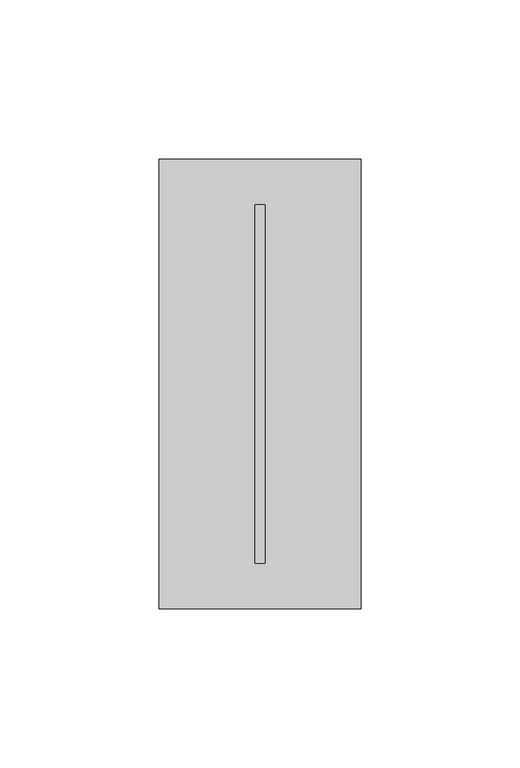
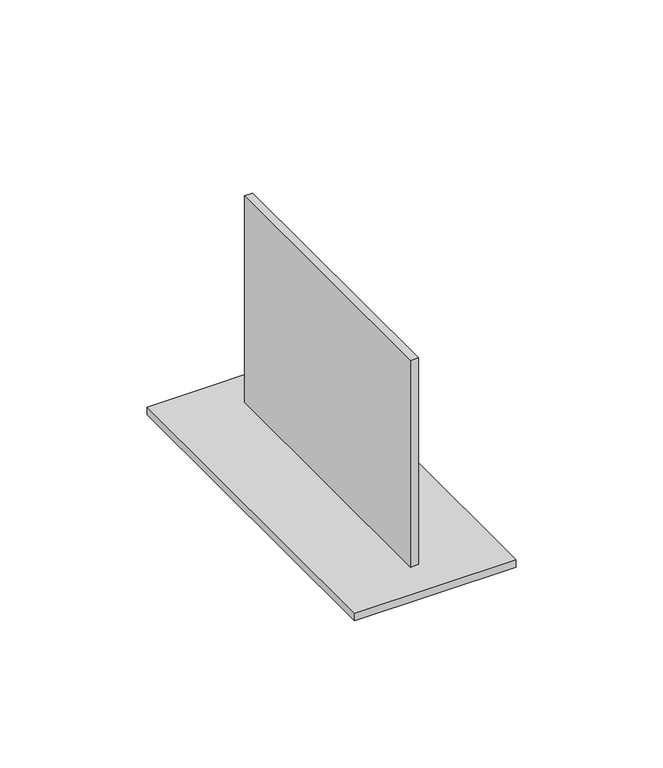
"""IFC4 building model written with IfcOpenShell, lengths in millimetres: proxy geometry, 060523 - W_P_C - Fastenings - Concealed Joist Ties : 060523 - W_P_C - Fastenings - Concealed Joist Ties."""

from ifc_helpers import new_model, si_unit, frame, origin, origin_with_axes, place, context, project, spatial, polyline, outline, extrude, source, transform, mapped, element, save


def generic_models_dea6e0a2(model_context):
    return source(origin(), model_context, "Body", "SweptSolid", [
        extrude(outline(polyline([(1.5875, -56.35625), (-1.5875, -56.35625), (-1.5875, 56.35625), (1.5875, 56.35625), (1.5875, -56.35625)])), frame((0.0, 0.0, 3.175), z_axis=(0.0, 0.0, 1.0), x_axis=(1.0, 0.0, 0.0)), (0.0, 0.0, 1.0), 85.725),
        extrude(outline(polyline([(31.75, -70.64375), (-31.75, -70.64375), (-31.75, 70.64375), (31.75, 70.64375), (31.75, -70.64375)])), origin_with_axes(), (0.0, 0.0, 1.0), 3.175),
    ])


if __name__ == "__main__":
    model = new_model("IFC4")
    model_context = context("Model", 3, world=origin())
    ifc_project = project(units=[si_unit("LENGTHUNIT", "METRE", prefix="MILLI")], contexts=[model_context])
    site = spatial("IfcSite", under=ifc_project)
    building = spatial("IfcBuilding", under=site)
    placement = place(None, origin())
    generic_models_shape = generic_models_dea6e0a2(model_context)
    element("IfcBuildingElementProxy", 1, Name="060523 - W_P_C - Fastenings - Concealed Joist Ties : 060523 - W_P_C - Fastenings - Concealed Joist Ties", ObjectType="060523 - W_P_C - Fastenings - Concealed Joist Ties : 060523 - W_P_C - Fastenings - Concealed Joist Ties", at=placement, inside=building, context=model_context, shape_type="MappedRepresentation", body=[
        mapped(generic_models_shape, transform((0.0, 0.0, 0.0), x_axis=(1.0, 0.0, 0.0), y_axis=(0.0, 1.0, 0.0), z_axis=(0.0, 0.0, 1.0))),
    ])
    save(model, "model.ifc")

# Revit data of these elements
# Type "060523 - W_P_C - Fastenings - Concealed Joist Ties : 060523 - W_P_C - Fastenings - Concealed Joist Ties"
#   OFFSET FROM SURFACE = 0' - 3"
#   H2 = 0' - 4 7/16"
#   H1 = 0' - 5 9/16"
#   GAUGE = 0' - 0 1/8"
#   Default Elevation = 4' - 0"
#   Material = _BEAM HANGER (SEE STRUCT. DWGS)
# Element 1 (IfcBuildingElementProxy, "060523 - W_P_C - Fastenings - Concealed Joist Ties : 060523 - W_P_C - Fastenings - Concealed Joist Ties")
#   Materials on its faces: "_BEAM HANGER (SEE STRUCT. DWGS)"
# Materials
#   "_BEAM HANGER (SEE STRUCT. DWGS)": class "Generic", colour RGB 191 191 191, transparency 0, Cost = 0
